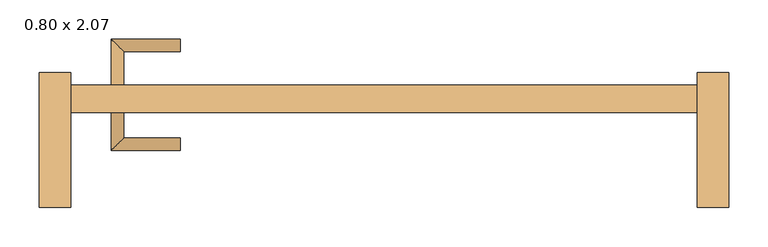
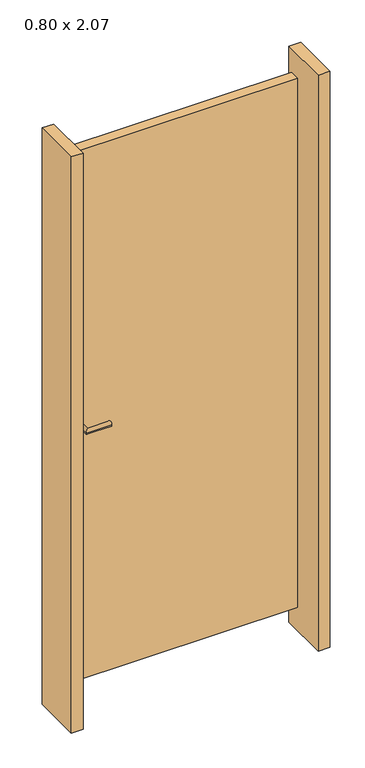
"""IFC4 building model written with IfcOpenShell, lengths in millimetres: door geometry, CC_ND 200_PORTÃO_V2018 : 0.80 x 2.07."""

from ifc_helpers import new_model, si_unit, frame, origin, origin_with_axes, place, context, project, spatial, polyline, circle_curve, ellipse_curve, outline, extrude, source, transform, mapped, element, save
from ifc_brep_helpers import plane_surface, cylinder_surface, advanced_brep


def door_0_80_x_2_07_c914aa4f(model_context):
    return source(origin(), model_context, "Body", "SolidModel", [
        advanced_brep(
        [(-348.0, 70.0, 1000.0), (-332.0, 70.0, 1000.0), (-348.0, 129.0, 1000.0), (-332.0, 113.0, 1000.0), (-260.0, 129.0, 1000.0), (-260.0, 113.0, 1000.0)],
        [
            (0, 1, circle_curve(frame((-340.0, 70.0, 1000.0), z_axis=(0.0, -1.0, 0.0), x_axis=(1.0, 0.0, 0.0)), 8.0)),
            (1, 0, circle_curve(frame((-340.0, 70.0, 1000.0), z_axis=(0.0, -1.0, 0.0), x_axis=(1.0, 0.0, 0.0)), 8.0)),
            (0, 2),
            (2, 3, ellipse_curve(frame((-340.0, 121.0, 1000.0), z_axis=(-0.707106781186538, -0.707106781186557, 0.0), x_axis=(0.707106781186557, -0.707106781186538, 0.0)), 11.3137085, 8.0)),
            (3, 1),
            (3, 2, ellipse_curve(frame((-340.0, 121.0, 1000.0), z_axis=(-0.707106781186538, -0.707106781186557, 0.0), x_axis=(0.707106781186557, -0.707106781186538, 0.0)), 11.3137085, 8.0)),
            (4, 5, circle_curve(frame((-260.0, 121.0, 1000.0), z_axis=(1.0, 0.0, 0.0), x_axis=(0.0, -1.0, 0.0)), 8.0)),
            (5, 4, circle_curve(frame((-260.0, 121.0, 1000.0), z_axis=(1.0, 0.0, 0.0), x_axis=(0.0, -1.0, 0.0)), 8.0)),
            (2, 4),
            (5, 3),
        ],
        [
            plane_surface(frame((-340.0, 70.0, 0.0), z_axis=(0.0, -1.0, 0.0), x_axis=(0.0, 0.0, 1.0))),
            cylinder_surface(frame((-340.0, 70.0, 1000.0), z_axis=(0.0, -1.0, 0.0), x_axis=(1.0, 0.0, 0.0)), 8.0),
            plane_surface(frame((-260.0, 121.0, 0.0), z_axis=(1.0, 0.0, 0.0), x_axis=(0.0, 0.0, 1.0))),
            cylinder_surface(frame((-340.0, 121.0, 1000.0), z_axis=(-1.0, 0.0, 0.0), x_axis=(0.0, -1.0, 0.0)), 8.0),
        ],
        [
            (0, [[1, 2]]),
            (1, [[3, 4, 5, -1]]),
            (1, [[-5, 6, -3, -2]]),
            (2, [[7, 8]]),
            (3, [[9, -8, 10, -4]]),
            (3, [[-10, -7, -9, -6]]),
        ],
    ),
        advanced_brep(
        [(-332.0, 35.0, 1000.0), (-348.0, 35.0, 1000.0), (-348.0, -13.0, 1000.0), (-332.0, 3.0, 1000.0), (-260.0, 3.0, 1000.0), (-260.0, -13.0, 1000.0)],
        [
            (0, 1, circle_curve(frame((-340.0, 35.0, 1000.0), z_axis=(0.0, 1.0, 0.0), x_axis=(-1.0, 0.0, 0.0)), 8.0)),
            (1, 0, circle_curve(frame((-340.0, 35.0, 1000.0), z_axis=(0.0, 1.0, 0.0), x_axis=(-1.0, 0.0, 0.0)), 8.0)),
            (1, 2),
            (2, 3, ellipse_curve(frame((-340.0, -5.0, 1000.0), z_axis=(-0.7071067811865475, 0.7071067811865475, 0.0), x_axis=(0.7071067811865474, 0.7071067811865476, 0.0)), 11.3137085, 8.0)),
            (3, 0),
            (3, 2, ellipse_curve(frame((-340.0, -5.0, 1000.0), z_axis=(-0.7071067811865475, 0.7071067811865475, 0.0), x_axis=(0.7071067811865474, 0.7071067811865476, 0.0)), 11.3137085, 8.0)),
            (4, 5, circle_curve(frame((-260.0, -5.0, 1000.0), z_axis=(1.0, 0.0, 0.0), x_axis=(0.0, -1.0, 0.0)), 8.0)),
            (5, 4, circle_curve(frame((-260.0, -5.0, 1000.0), z_axis=(1.0, 0.0, 0.0), x_axis=(0.0, -1.0, 0.0)), 8.0)),
            (2, 5),
            (4, 3),
        ],
        [
            plane_surface(frame((-340.0, 35.0, 0.0), z_axis=(0.0, 1.0, 0.0), x_axis=(0.0, 0.0, 1.0))),
            cylinder_surface(frame((-340.0, 35.0, 1000.0), z_axis=(0.0, 1.0, 0.0), x_axis=(-1.0, 0.0, 0.0)), 8.0),
            plane_surface(frame((-260.0, -5.0, 0.0), z_axis=(1.0, 0.0, 0.0), x_axis=(0.0, 0.0, 1.0))),
            cylinder_surface(frame((-340.0, -5.0, 1000.0), z_axis=(-1.0, 0.0, 0.0), x_axis=(0.0, -1.0, 0.0)), 8.0),
        ],
        [
            (0, [[1, 2]]),
            (1, [[3, 4, 5, -2]]),
            (1, [[-5, 6, -3, -1]]),
            (2, [[7, 8]]),
            (3, [[9, -7, 10, -4]]),
            (3, [[-10, -8, -9, -6]]),
        ],
    ),
        extrude(outline(polyline([(400.0, 70.0), (400.0, 35.0), (-400.0, 35.0), (-400.0, 70.0), (400.0, 70.0)])), frame((0.0, 0.0, 85.0), z_axis=(0.0, 0.0, 1.0), x_axis=(1.0, 0.0, 0.0)), (0.0, 0.0, 1.0), 1900.0),
        extrude(outline(polyline([(-440.0, -86.0), (-440.0, 86.0), (-400.0, 86.0), (-400.0, -86.0), (-440.0, -86.0)])), origin_with_axes(), (0.0, 0.0, 1.0), 2070.0),
        extrude(outline(polyline([(440.0, -86.0), (400.0, -86.0), (400.0, 86.0), (440.0, 86.0), (440.0, -86.0)])), origin_with_axes(), (0.0, 0.0, 1.0), 2070.0),
    ])


if __name__ == "__main__":
    model = new_model("IFC4")
    model_context = context("Model", 3, world=origin())
    ifc_project = project(units=[si_unit("LENGTHUNIT", "METRE", prefix="MILLI")], contexts=[model_context])
    site = spatial("IfcSite", under=ifc_project)
    building = spatial("IfcBuilding", under=site)
    placement = place(None, origin())
    door_0_80_x_2_07_shape = door_0_80_x_2_07_c914aa4f(model_context)
    element("IfcDoor", 1, ObjectType="CC_ND 200_PORTÃO_V2018 : 0.80 x 2.07", at=placement, inside=building, context=model_context, shape_type="MappedRepresentation", body=[
        mapped(door_0_80_x_2_07_shape, transform((0.0, 0.0, 0.0), x_axis=(1.0, 0.0, 0.0), y_axis=(0.0, 1.0, 0.0), z_axis=(0.0, 0.0, 1.0))),
    ])
    save(model, "model.ifc")

# Revit data of these elements
# Type "CC_ND 200_PORTÃO_V2018 : 0.80 x 2.07"
#   Type Mark = "141"
#   Analytic Construction = "<Nenhum>"
#   Vão superior = 0.085 m
#   Vão inferior = 0.085 m
#   Largura_moldura = 0.08 m
#   Espessura_moldura = 0.01 m
#   Espessura_batente = 0.04 m
#   Thickness = 0.05 m
#   Altura do portão = 1.90 m
#   Rough Width = 0.88 m
#   Rough Height = 1.73 m
#   Height = 1.73 m
#   Width = 0.80 m
#   Soleira [instance default] = no
#   Moldura_interna [instance default] = no
#   Moldura_externa [instance default] = no
#   Maçaneta [instance default] = no
#   Acabamento moldura [instance default] = none
#   Acabamento batente [instance default] = none
#   Acabamento maçaneta [instance default] = none
#   Acabamento folha da porta [instance default] = none
#   Acabamento soleira [instance default] = none
#   Function = (empty or 0)
#   Wall Closure = (empty or 0)
# Element 1 (IfcDoor, "CC_ND 200_PORTÃO_V2018 : 0.80 x 2.07")
#   Maçaneta = yes
#   Acabamento moldura = .ALUMÍNIO
#   Acabamento batente = .MADEIRA_CEREJEIRA CLARO
#   Acabamento folha da porta = .MADEIRA_CEREJEIRA CLARO
#   Materials on its faces: ".MADEIRA_CEREJEIRA CLARO"
# Materials
#   ".MADEIRA_CEREJEIRA CLARO": class ".CC_MADEIRA REVEST.", colour RGB 233 182 144, transparency 0, Cost = 0
#   ".ALUMÍNIO": class "CC_METAIS", colour RGB 244 244 244, transparency 0, Description = "Material alumínio", Cost = 0
